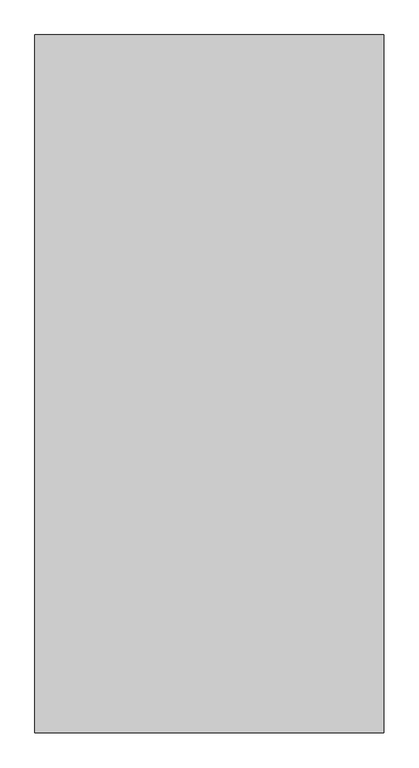
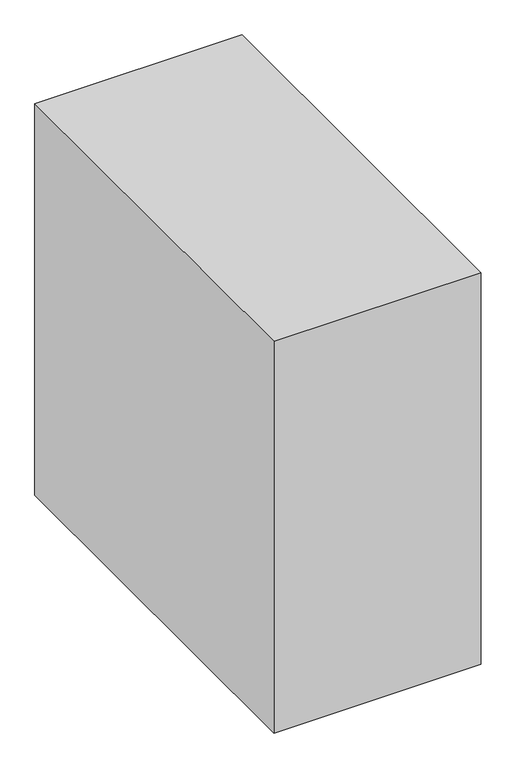
"""IFC4 building model written with IfcOpenShell, lengths in millimetres: proxy geometry, Space Planning Box_hec : Space Planning Box_hec."""

import ifcopenshell
import ifcopenshell.guid

model = None  # the IFC model being written
_history = None  # IfcOwnerHistory: only IFC2X3 demands one
_inside = {}  # id of a spatial element -> (the spatial element, [elements in it])
_under = {}  # id of a project, library or spatial element -> (it, [spatial elements below it])
_declared = {}  # id of a project -> (the project, [libraries it declares])
_typed = {}  # id of a type object -> (the type object, [elements of that type])
_made_of = {}  # id of a material, layer set ... -> (it, [elements and type objects made of it])


def new_model(schema):
    """Start an empty IFC model of exactly this schema.

    Asked for "IFC4X3", IfcOpenShell would pick the latest addendum, in which some entities
    have other attributes; the version numbers below select the first issue.
    IFC2X3 requires an IfcOwnerHistory on every rooted entity: one is made here for all.
    """
    global model, _history
    if schema == "IFC4X3":
        model = ifcopenshell.file(schema_version=(4, 3, 0, 0))
    else:
        model = ifcopenshell.file(schema=schema)
    _inside.clear()
    _under.clear()
    _declared.clear()
    _typed.clear()
    _made_of.clear()
    _history = None
    if model.schema == "IFC2X3":
        org = make("IfcOrganization", Name="unknown")
        user = make(
            "IfcPersonAndOrganization",
            ThePerson=make("IfcPerson", FamilyName="unknown"),
            TheOrganization=org,
        )
        app = make(
            "IfcApplication",
            ApplicationDeveloper=org,
            Version="unknown",
            ApplicationFullName="unknown",
            ApplicationIdentifier="unknown",
        )
        _history = make(
            "IfcOwnerHistory",
            OwningUser=user,
            OwningApplication=app,
            ChangeAction="ADDED",
            CreationDate=0,
        )
    return model


def make(cls, **values):
    """One entity of the class cls with the attributes given. An attribute that is None is left unset."""
    return model.create_entity(
        cls, **{name: value for name, value in values.items() if value is not None}
    )


def rooted(cls, **values):
    """An entity with a GlobalId (a new one), such as an element, a storey or a relation."""
    return make(cls, GlobalId=ifcopenshell.guid.new(), OwnerHistory=_history, **values)


def si_unit(unit_type, name, prefix=None):
    """IfcSIUnit, for example si_unit("LENGTHUNIT", "METRE", prefix="MILLI")."""
    return make("IfcSIUnit", UnitType=unit_type, Prefix=prefix, Name=name)


def assignment(units):
    """IfcUnitAssignment: the units of a project."""
    return None if units is None else make("IfcUnitAssignment", Units=units)


def point(xyz):
    """IfcCartesianPoint."""
    return None if xyz is None else make("IfcCartesianPoint", Coordinates=xyz)


def direction(xyz):
    """IfcDirection."""
    return None if xyz is None else make("IfcDirection", DirectionRatios=xyz)


def frame(location, z_axis=None, x_axis=None):
    """IfcAxis2Placement3D, a coordinate frame: its origin and axes. An axis left out is left unset."""
    return make(
        "IfcAxis2Placement3D",
        Location=point(location),
        Axis=direction(z_axis),
        RefDirection=direction(x_axis),
    )


def origin():
    """The frame at (0, 0, 0) with its axes left unset."""
    return frame((0.0, 0.0, 0.0))


def origin_with_axes():
    """The frame at (0, 0, 0) with the z axis (0, 0, 1) and the x axis (1, 0, 0) written out."""
    return frame((0.0, 0.0, 0.0), z_axis=(0.0, 0.0, 1.0), x_axis=(1.0, 0.0, 0.0))


def place(relative_to, where):
    """IfcLocalPlacement: puts the frame where relative to a parent placement (None: the world)."""
    return make(
        "IfcLocalPlacement", PlacementRelTo=relative_to, RelativePlacement=where
    )


def context(
    kind, dimensions, precision=None, world=None, true_north=None, identifier=None
):
    """IfcGeometricRepresentationContext, for example the 3D "Model" context."""
    return make(
        "IfcGeometricRepresentationContext",
        ContextIdentifier=identifier,
        ContextType=kind,
        CoordinateSpaceDimension=dimensions,
        Precision=precision,
        WorldCoordinateSystem=world,
        TrueNorth=true_north,
    )


def project(units=None, contexts=None):
    """IfcProject with its units and contexts."""
    return rooted(
        "IfcProject",
        Name="project",
        RepresentationContexts=contexts,
        UnitsInContext=assignment(units),
    )


def spatial(cls, under=None, at=None, **own):
    """A site, building, storey or space (cls), placed at a placement, below another one or the project."""
    s = rooted(cls, ObjectPlacement=at, **own)
    if under is not None:
        _under.setdefault(under.id(), (under, []))[1].append(s)
    return s


def polyline(points):
    """IfcPolyline through the points."""
    return make("IfcPolyline", Points=[point(p) for p in points])


def outline(outer, holes=None, kind="AREA"):
    """IfcArbitraryClosedProfileDef: a profile drawn as a closed curve; with holes, ...WithVoids."""
    if holes is None:
        return make("IfcArbitraryClosedProfileDef", ProfileType=kind, OuterCurve=outer)
    return make(
        "IfcArbitraryProfileDefWithVoids",
        ProfileType=kind,
        OuterCurve=outer,
        InnerCurves=holes,
    )


def extrude(swept, where, along, depth):
    """IfcExtrudedAreaSolid: the profile swept, set in the frame where, extruded along a direction by depth."""
    return make(
        "IfcExtrudedAreaSolid",
        SweptArea=swept,
        Position=where,
        ExtrudedDirection=direction(along),
        Depth=depth,
    )


def shape(context_of_items, identifier, shape_type, items):
    """IfcShapeRepresentation: the items that make up one representation, for example the "Body"."""
    return make(
        "IfcShapeRepresentation",
        ContextOfItems=context_of_items,
        RepresentationIdentifier=identifier,
        RepresentationType=shape_type,
        Items=items,
    )


def source(mapping_origin, context_of_items, identifier, shape_type, items):
    """IfcRepresentationMap: a shape defined once, which mapped items show again and again."""
    return make(
        "IfcRepresentationMap",
        MappingOrigin=mapping_origin,
        MappedRepresentation=shape(context_of_items, identifier, shape_type, items),
    )


def transform(
    local_origin,
    x_axis=None,
    y_axis=None,
    z_axis=None,
    scale=None,
    scale2=None,
    scale3=None,
    uniform=True,
):
    """IfcCartesianTransformationOperator3D, or its non-uniform kind. x_axis, y_axis, z_axis: its Axis1, 2, 3."""
    if uniform:
        return make(
            "IfcCartesianTransformationOperator3D",
            Axis1=direction(x_axis),
            Axis2=direction(y_axis),
            LocalOrigin=point(local_origin),
            Scale=scale,
            Axis3=direction(z_axis),
        )
    return make(
        "IfcCartesianTransformationOperator3DnonUniform",
        Axis1=direction(x_axis),
        Axis2=direction(y_axis),
        LocalOrigin=point(local_origin),
        Scale=scale,
        Axis3=direction(z_axis),
        Scale2=scale2,
        Scale3=scale3,
    )


def mapped(mapping_source, mapping_target):
    """IfcMappedItem: shows the shape of a source again, moved by a transform."""
    return make(
        "IfcMappedItem", MappingSource=mapping_source, MappingTarget=mapping_target
    )


def made_of(thing, what):
    """Note that an element or type object is made of a material, layer set ...; save() writes the relation."""
    if what is not None:
        _made_of.setdefault(what.id(), (what, []))[1].append(thing)
    return thing


def element(
    cls,
    number,
    at=None,
    inside=None,
    cuts=None,
    type_object=None,
    material=None,
    context=None,
    identifier="Body",
    shape_type=None,
    held_by="IfcProductDefinitionShape",
    body=None,
    shapes=None,
    **own,
):
    """One element of the class cls, such as IfcWall. Its Tag is "e" and its number.

    at: its placement. inside: the storey or other place that contains it. cuts: it is an
    opening in that element (IfcRelVoidsElement). A single representation is given by context,
    identifier, shape_type and body (its items); several are given by shapes. held_by: the class
    of the entity that holds the representations. save() writes the other relations.
    """
    e = rooted(cls, Tag="e%d" % number, ObjectPlacement=at, **own)
    if body is not None:
        shapes = [shape(context, identifier, shape_type, body)]
    if shapes is not None:
        e.Representation = make(held_by, Representations=shapes)
    if inside is not None:
        _inside.setdefault(inside.id(), (inside, []))[1].append(e)
    if cuts is not None:
        rooted(
            "IfcRelVoidsElement", RelatingBuildingElement=cuts, RelatedOpeningElement=e
        )
    if type_object is not None:
        _typed.setdefault(type_object.id(), (type_object, []))[1].append(e)
    return made_of(e, material)


def aggregate(whole, parts):
    """IfcRelAggregates: a whole, such as a stair, and the parts it consists of."""
    return rooted("IfcRelAggregates", RelatingObject=whole, RelatedObjects=parts)


def save(model, path):
    """Write the relations noted so far, then the file.

    IfcRelAggregates (storeys below a building ...), IfcRelContainedInSpatialStructure (elements
    in a storey), IfcRelDefinesByType, IfcRelAssociatesMaterial and IfcRelDeclares: one each for
    every whole, place, type object, material and project.
    """
    for whole, parts in _under.values():
        aggregate(whole, parts)
    for where, things in _inside.values():
        rooted(
            "IfcRelContainedInSpatialStructure",
            RelatedElements=things,
            RelatingStructure=where,
        )
    for kind, things in _typed.values():
        rooted("IfcRelDefinesByType", RelatedObjects=things, RelatingType=kind)
    for what, things in _made_of.values():
        rooted("IfcRelAssociatesMaterial", RelatedObjects=things, RelatingMaterial=what)
    for by, libraries in _declared.values():
        rooted("IfcRelDeclares", RelatingContext=by, RelatedDefinitions=libraries)
    model.write(path)


def generic_models_542cc789(model_context):
    return source(origin(), model_context, "Body", "SweptSolid", [
        extrude(outline(polyline([(1500.0, 3000.0), (1500.0, -3000.0), (-1500.0, -3000.0), (-1500.0, 3000.0), (1500.0, 3000.0)])), origin_with_axes(), (0.0, 0.0, 1.0), 6000.0),
    ])


if __name__ == "__main__":
    model = new_model("IFC4")
    model_context = context("Model", 3, world=origin())
    ifc_project = project(units=[si_unit("LENGTHUNIT", "METRE", prefix="MILLI")], contexts=[model_context])
    site = spatial("IfcSite", under=ifc_project)
    building = spatial("IfcBuilding", under=site)
    placement = place(None, origin())
    generic_models_shape = generic_models_542cc789(model_context)
    element("IfcBuildingElementProxy", 1, Name="Space Planning Box_hec : Space Planning Box_hec", ObjectType="Space Planning Box_hec : Space Planning Box_hec", at=placement, inside=building, context=model_context, shape_type="MappedRepresentation", body=[
        mapped(generic_models_shape, transform((0.0, 0.0, 0.0), x_axis=(1.0, 0.0, 0.0), y_axis=(0.0, 1.0, 0.0), z_axis=(0.0, 0.0, 1.0))),
    ])
    save(model, "model.ifc")

# Revit data of these elements
# Type "Space Planning Box_hec : Space Planning Box_hec"
#   Type Comments = "..."
#   Room Name [instance default] = "?"
#   Interior Finish [instance default] = ""
#   Exterior Finish [instance default] = ""
#   Department [instance default] = ""
#   Assembly Code = "..."
#   Width [instance default] = 1524 mm
#   Program Area [instance default] = 0.00 m²
#   Length [instance default] = 1524 mm
#   Height [instance default] = 1524 mm
#   Area [instance default] = 2.32258 m²
#   Fill Color [instance default] = Cyan
#   Default Elevation = 0
# Element 1 (IfcBuildingElementProxy, "Space Planning Box_hec : Space Planning Box_hec")
#   Room Name = "LOTO Office Room"
#   Interior Finish = "IF2-1"
#   Exterior Finish = "EF1"
#   Department = "AR"
#   Width = 3000 mm
#   Program Area = 31.50 m²
#   Length = 6000 mm
#   Height = 6000 mm
#   Area = 18.00 m²
#   Fill Color = Lavender
#   Materials on its faces: "Lavender"
# Materials
#   "Cyan": class "Generic", colour RGB 0 255 255, transparency 0.2, Cost = 0
#   "Lavender": class "Generic", colour RGB 186 85 211, transparency 0.2, Cost = 0
